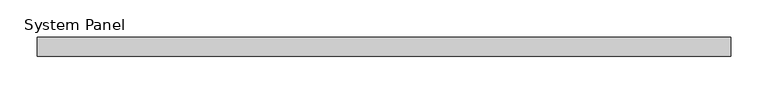
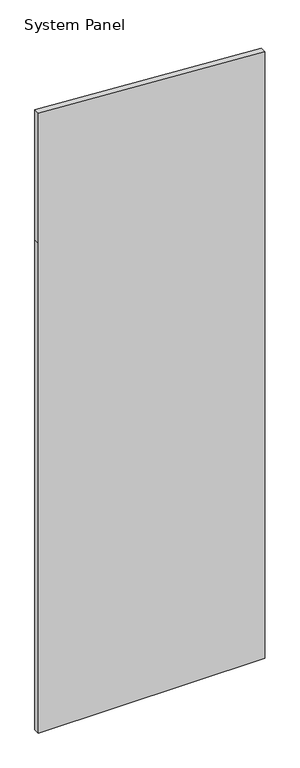
"""IFC4 building model written with IfcOpenShell, lengths in millimetres: plate geometry, System Panel : TEMPERED INSULATED GLAZING (CARDINAL GLASS LoĒ²-240."""

from ifc_helpers import new_model, si_unit, frame, origin, place, context, project, spatial, polyline, outline, extrude, source, transform, mapped, element, save


def system_panel_b414e7e6(model_context):
    return source(origin(), model_context, "Body", "SweptSolid", [
        extrude(outline(polyline([(0.0, -464.740625), (0.0, 464.740625), (2127.25, 464.740625), (2633.7122061, 464.740625), (2691.8047842, -464.740625), (2127.25, -464.740625), (0.0, -464.740625)])), frame((0.0, 6.35, 0.0), z_axis=(0.0, 1.0, 0.0), x_axis=(0.0, 0.0, 1.0)), (0.0, 0.0, 1.0), 25.4),
    ])


if __name__ == "__main__":
    model = new_model("IFC4")
    model_context = context("Model", 3, world=origin())
    ifc_project = project(units=[si_unit("LENGTHUNIT", "METRE", prefix="MILLI")], contexts=[model_context])
    site = spatial("IfcSite", under=ifc_project)
    building = spatial("IfcBuilding", under=site)
    placement = place(None, origin())
    system_panel_shape = system_panel_b414e7e6(model_context)
    element("IfcPlate", 1, ObjectType="System Panel : TEMPERED INSULATED GLAZING (CARDINAL GLASS LoĒ²-240", at=placement, inside=building, context=model_context, shape_type="MappedRepresentation", body=[
        mapped(system_panel_shape, transform((0.0, 0.0, 0.0), x_axis=(1.0, 0.0, 0.0), y_axis=(0.0, 1.0, 0.0), z_axis=(0.0, 0.0, 1.0))),
    ])
    save(model, "model.ifc")

# Revit data of these elements
# Type "System Panel : TEMPERED INSULATED GLAZING (CARDINAL GLASS LoĒ²-240"
#   Construction Type Id = "opn-s72"
#   Analytic Construction = "Double glazing - 1/4 in thick - low-E/clear (e = 0.1) glass"
#   Visual Light Transmittance = 0.72
#   Solar Heat Gain Coefficient = 0.6
#   Heat Transfer Coefficient (U) = 1.9873 W/(m²·K)
#   Transparency_Hack = 70
# Element 1 (IfcPlate, "System Panel : TEMPERED INSULATED GLAZING (CARDINAL GLASS LoĒ²-240")
#   Materials on its faces: "TEMPERED INSULATED GLAZING (CARDINAL GLASS LoĒ²-240\nOR EQUIVALENT)"
# Materials
#   "TEMPERED INSULATED GLAZING (CARDINAL GLASS LoĒ²-240\nOR EQUIVALENT)": class "Glass", colour RGB 196 205 210, transparency 0.85, Description = "Soda Lime Glass", Cost = 0
